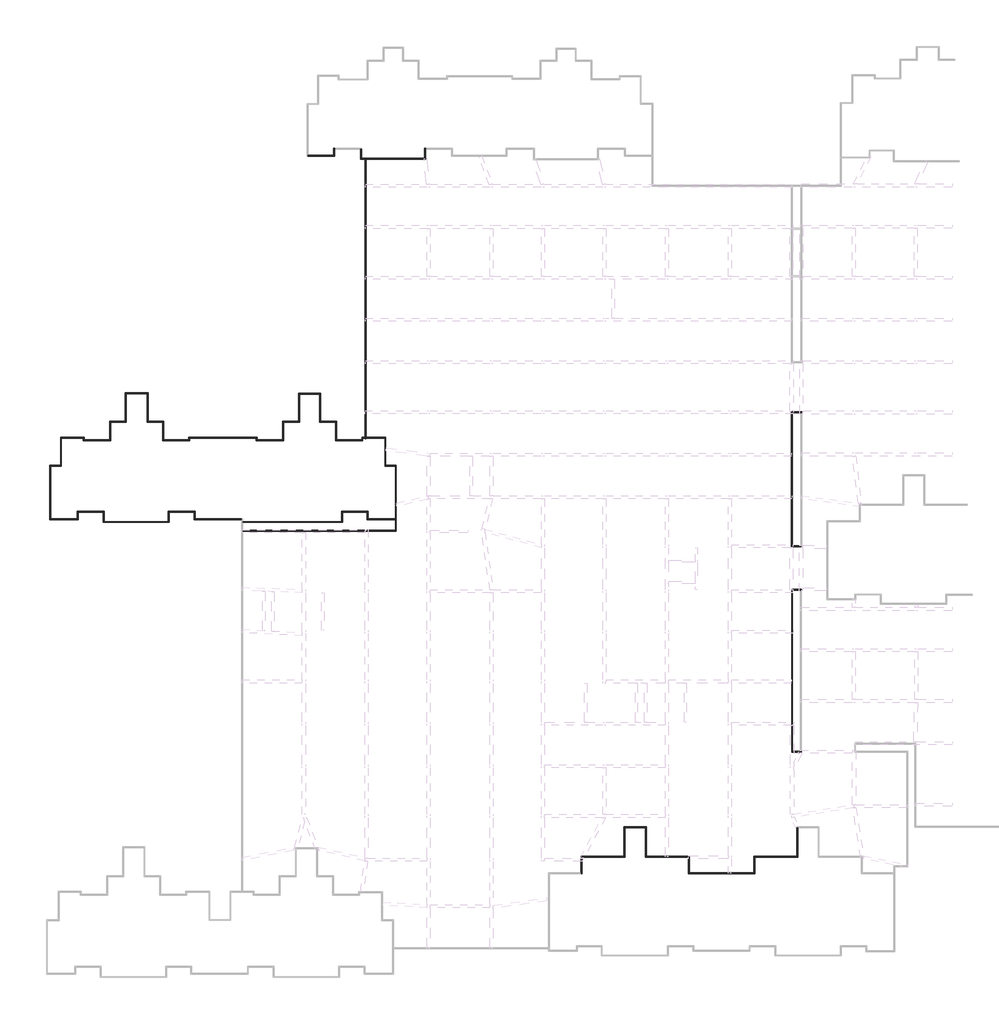
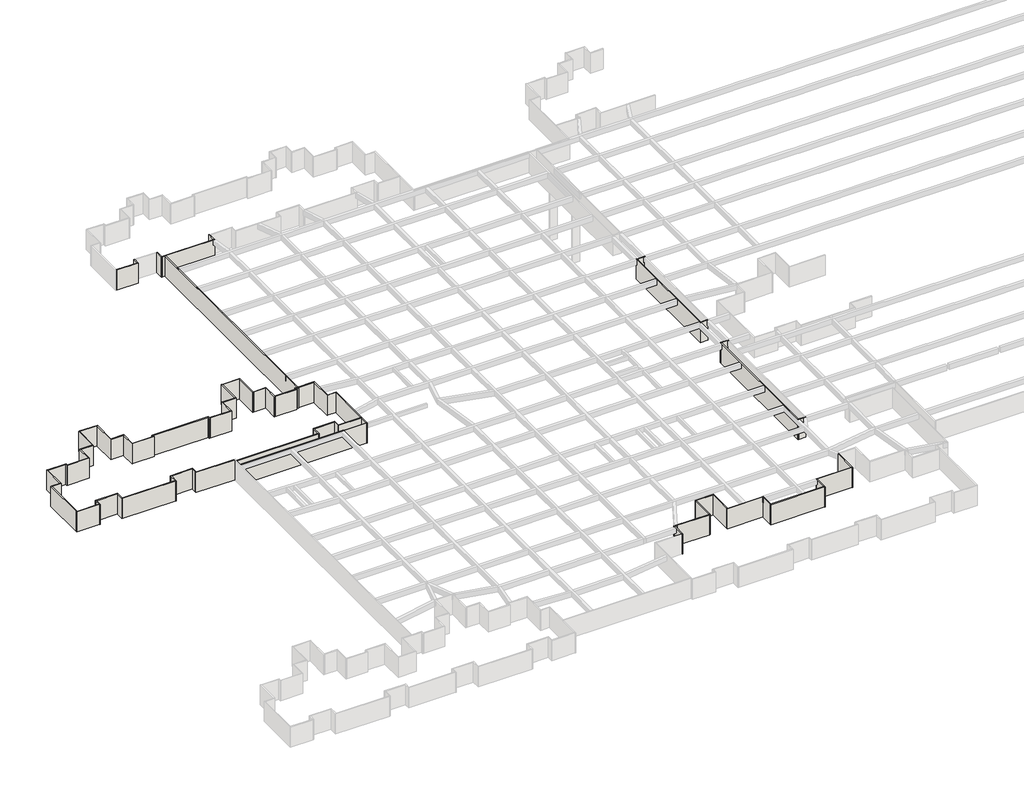
# One storey, part 2 of 16: 69 walls.
"""IFC4 building model written with IfcOpenShell, lengths in millimetres."""

from ifc_helpers import new_model, si_unit, origin, origin_with_axes, place, context, project, spatial, polyline, outline, extrude, faceted_brep, element, save

model = new_model("IFC4")

# Units and contexts
model_context = context("Model", 3, world=origin())
ifc_project = project(units=[si_unit("LENGTHUNIT", "METRE", prefix="MILLI")], contexts=[model_context])

# Site, building, storey
site = spatial("IfcSite", under=ifc_project)
building = spatial("IfcBuilding", under=site)
storey = spatial("IfcBuildingStorey", under=building, Name="户型图", Elevation=0.0)

# Walls
placement = place(None, origin())
element("IfcWall", 1, ObjectType="所有墙体", at=placement, inside=storey, context=model_context, shape_type="Brep", body=[
    faceted_brep([(192826.317546, -128736.151487, 0.0), (196226.317546, -128736.151487, 0.0), (196226.317546, -128736.151487, 3300.0), (192826.317546, -128736.151487, 3300.0), (192826.317546, -128616.151487, 0.0), (192826.317546, -128616.151487, 3300.0), (196106.317546, -128616.151487, 3300.0), (196226.317546, -128616.151487, 3300.0), (196226.317546, -128616.151487, 0.0), (196106.317546, -128616.151487, 0.0)], [[[0, 1, 2, 3]], [[4, 5, 6, 7, 8, 9]], [[1, 0, 4, 9, 8]], [[3, 2, 7, 6, 5]], [[0, 3, 5, 4]], [[2, 1, 8, 7]]]),
])
element("IfcWall", 2, ObjectType="所有墙体", at=placement, inside=storey, context=model_context, shape_type="Brep", body=[
    faceted_brep([(196226.317546, -128616.151487, 0.0), (196226.317546, -127836.151487, 0.0), (196226.317546, -127716.151487, 0.0), (196226.317546, -127716.151487, 3300.0), (196226.317546, -127836.151487, 3300.0), (196226.317546, -128616.151487, 3300.0), (196106.317546, -128616.151487, 0.0), (196106.317546, -128616.151487, 3300.0), (196106.317546, -127716.151487, 3300.0), (196106.317546, -127716.151487, 0.0)], [[[0, 1, 2, 3, 4, 5]], [[6, 7, 8, 9]], [[2, 1, 0, 6, 9]], [[5, 4, 3, 8, 7]], [[0, 5, 7, 6]], [[3, 2, 9, 8]]]),
])
element("IfcWall", 3, ObjectType="所有墙体", at=placement, inside=storey, context=model_context, shape_type="Brep", body=[
    faceted_brep([(199599.9062186, -127836.151487, 0.0), (199599.9062186, -129094.6769035, 0.0), (199599.9062186, -129094.6769035, 3300.0), (199599.9062186, -127836.151487, 3300.0), (199719.9062186, -127836.151487, 0.0), (199719.9062186, -127836.151487, 3300.0), (199719.9062186, -128974.6769035, 3300.0), (199719.9062186, -129094.6769035, 3300.0), (199719.9062186, -129094.6769035, 0.0), (199719.9062186, -128974.6769035, 0.0)], [[[0, 1, 2, 3]], [[4, 5, 6, 7, 8, 9]], [[1, 0, 4, 9, 8]], [[3, 2, 7, 6, 5]], [[0, 3, 5, 4]], [[2, 1, 8, 7]]]),
])
element("IfcWall", 4, ObjectType="所有墙体", at=placement, inside=storey, context=model_context, shape_type="Brep", body=[
    faceted_brep([(199719.9062186, -129094.6769035, 0.0), (200143.757676, -129094.6769035, 0.0), (200263.757676, -129094.6769035, 0.0), (207918.5069416, -129094.6769035, 0.0), (207918.5069416, -129094.6769035, 3300.0), (200263.757676, -129094.6769035, 3300.0), (200143.757676, -129094.6769035, 3300.0), (199719.9062186, -129094.6769035, 3300.0), (199719.9062186, -128974.6769035, 0.0), (199719.9062186, -128974.6769035, 3300.0), (207798.5069416, -128974.6769035, 3300.0), (207918.5069416, -128974.6769035, 3300.0), (207918.5069416, -128974.6769035, 0.0), (207798.5069416, -128974.6769035, 0.0)], [[[0, 1, 2, 3, 4, 5, 6, 7]], [[8, 9, 10, 11, 12, 13]], [[3, 2, 1, 0, 8, 13, 12]], [[7, 6, 5, 4, 11, 10, 9]], [[0, 7, 9, 8]], [[4, 3, 12, 11]]]),
])
element("IfcWall", 5, ObjectType="所有墙体", at=placement, inside=storey, context=model_context, shape_type="SweptSolid", body=[
    extrude(outline(polyline([(200143.757676, -165025.7214763), (200143.757676, -129094.6769035), (200263.757676, -129094.6769035), (200263.757676, -165025.7214763), (200143.757676, -165025.7214763)])), origin_with_axes(), (0.0, 0.0, 1.0), 3300.0),
])
element("IfcWall", 6, ObjectType="所有墙体", at=placement, inside=storey, context=model_context, shape_type="Brep", body=[
    faceted_brep([(207918.5069416, -128974.6769035, 0.0), (207918.5069416, -127836.151487, 0.0), (207918.5069416, -127716.151487, 0.0), (207918.5069416, -127716.151487, 3300.0), (207918.5069416, -127836.151487, 3300.0), (207918.5069416, -128974.6769035, 3300.0), (207798.5069416, -128974.6769035, 0.0), (207798.5069416, -128974.6769035, 3300.0), (207798.5069416, -127716.151487, 3300.0), (207798.5069416, -127716.151487, 0.0)], [[[0, 1, 2, 3, 4, 5]], [[6, 7, 8, 9]], [[2, 1, 0, 6, 9]], [[5, 4, 3, 8, 7]], [[0, 5, 7, 6]], [[3, 2, 9, 8]]]),
])
element("IfcWall", 7, ObjectType="所有墙体", at=placement, inside=storey, context=model_context, shape_type="Brep", body=[
    faceted_brep([(255612.4739458, -214925.8350287, 0.0), (255612.4739458, -218613.6358224, 0.0), (255612.4739458, -218733.6358224, 0.0), (255612.4739458, -218733.6358224, 3300.0), (255612.4739458, -218613.6358224, 3300.0), (255612.4739458, -214925.8350287, 3300.0), (255732.4739458, -214925.8350287, 0.0), (255732.4739458, -214925.8350287, 3300.0), (255732.4739458, -218733.6358224, 3300.0), (255732.4739458, -218733.6358224, 0.0)], [[[0, 1, 2, 3, 4, 5]], [[6, 7, 8, 9]], [[2, 1, 0, 6, 9]], [[5, 4, 3, 8, 7]], [[0, 5, 7, 6]], [[3, 2, 9, 8]]]),
])
element("IfcWall", 8, ObjectType="所有墙体", at=placement, inside=storey, context=model_context, shape_type="Brep", body=[
    faceted_brep([(255612.4739458, -218613.6358224, 0.0), (250108.5691963, -218613.6358224, 0.0), (250108.5691963, -218613.6358224, 3300.0), (255612.4739458, -218613.6358224, 3300.0), (255612.4739458, -218733.6358224, 0.0), (255612.4739458, -218733.6358224, 3300.0), (250228.5691963, -218733.6358224, 3300.0), (250108.5691963, -218733.6358224, 3300.0), (250108.5691963, -218733.6358224, 0.0), (250228.5691963, -218733.6358224, 0.0)], [[[0, 1, 2, 3]], [[4, 5, 6, 7, 8, 9]], [[1, 0, 4, 9, 8]], [[3, 2, 7, 6, 5]], [[0, 3, 5, 4]], [[2, 1, 8, 7]]]),
])
element("IfcWall", 9, ObjectType="所有墙体", at=placement, inside=storey, context=model_context, shape_type="Brep", body=[
    faceted_brep([(250108.5691963, -218733.6358224, 0.0), (250108.5691963, -220713.7545432, 0.0), (250108.5691963, -220833.7545432, 0.0), (250108.5691963, -220833.7545432, 3300.0), (250108.5691963, -220713.7545432, 3300.0), (250108.5691963, -218733.6358224, 3300.0), (250228.5691963, -218733.6358224, 0.0), (250228.5691963, -218733.6358224, 3300.0), (250228.5691963, -220833.7545432, 3300.0), (250228.5691963, -220833.7545432, 0.0)], [[[0, 1, 2, 3, 4, 5]], [[6, 7, 8, 9]], [[2, 1, 0, 6, 9]], [[5, 4, 3, 8, 7]], [[0, 5, 7, 6]], [[3, 2, 9, 8]]]),
])
element("IfcWall", 10, ObjectType="所有墙体", at=placement, inside=storey, context=model_context, shape_type="Brep", body=[
    faceted_brep([(250108.5691963, -220713.7545432, 0.0), (241826.9885063, -220713.7545432, 0.0), (241706.9885063, -220713.7545432, 0.0), (241706.9885063, -220713.7545432, 3300.0), (241826.9885063, -220713.7545432, 3300.0), (250108.5691963, -220713.7545432, 3300.0), (250108.5691963, -220833.7545432, 0.0), (250108.5691963, -220833.7545432, 3300.0), (241706.9885063, -220833.7545432, 3300.0), (241706.9885063, -220833.7545432, 0.0)], [[[0, 1, 2, 3, 4, 5]], [[6, 7, 8, 9]], [[2, 1, 0, 6, 9]], [[5, 4, 3, 8, 7]], [[0, 5, 7, 6]], [[3, 2, 9, 8]]]),
])
element("IfcWall", 11, ObjectType="所有墙体", at=placement, inside=storey, context=model_context, shape_type="Brep", body=[
    faceted_brep([(241826.9885063, -220713.7545432, 0.0), (241826.9885063, -218613.6358224, 0.0), (241826.9885063, -218613.6358224, 3300.0), (241826.9885063, -220713.7545432, 3300.0), (241706.9885063, -220713.7545432, 0.0), (241706.9885063, -220713.7545432, 3300.0), (241706.9885063, -218733.6358224, 3300.0), (241706.9885063, -218613.6358224, 3300.0), (241706.9885063, -218613.6358224, 0.0), (241706.9885063, -218733.6358224, 0.0)], [[[0, 1, 2, 3]], [[4, 5, 6, 7, 8, 9]], [[1, 0, 4, 9, 8]], [[3, 2, 7, 6, 5]], [[0, 3, 5, 4]], [[2, 1, 8, 7]]]),
])
element("IfcWall", 12, ObjectType="所有墙体", at=placement, inside=storey, context=model_context, shape_type="Brep", body=[
    faceted_brep([(241706.9885063, -218613.6358224, 0.0), (236279.3285625, -218613.6358224, 0.0), (236159.3285625, -218613.6358224, 0.0), (236159.3285625, -218613.6358224, 3300.0), (236279.3285625, -218613.6358224, 3300.0), (241706.9885063, -218613.6358224, 3300.0), (241706.9885063, -218733.6358224, 0.0), (241706.9885063, -218733.6358224, 3300.0), (236159.3285625, -218733.6358224, 3300.0), (236159.3285625, -218733.6358224, 0.0)], [[[0, 1, 2, 3, 4, 5]], [[6, 7, 8, 9]], [[2, 1, 0, 6, 9]], [[5, 4, 3, 8, 7]], [[0, 5, 7, 6]], [[3, 2, 9, 8]]]),
])
element("IfcWall", 13, ObjectType="所有墙体", at=placement, inside=storey, context=model_context, shape_type="Brep", body=[
    faceted_brep([(236279.3285625, -218613.6358224, 0.0), (236279.3285625, -214805.8350287, 0.0), (236279.3285625, -214805.8350287, 3300.0), (236279.3285625, -218613.6358224, 3300.0), (236159.3285625, -218613.6358224, 0.0), (236159.3285625, -218613.6358224, 3300.0), (236159.3285625, -214925.8350287, 3300.0), (236159.3285625, -214805.8350287, 3300.0), (236159.3285625, -214805.8350287, 0.0), (236159.3285625, -214925.8350287, 0.0)], [[[0, 1, 2, 3]], [[4, 5, 6, 7, 8, 9]], [[1, 0, 4, 9, 8]], [[3, 2, 7, 6, 5]], [[0, 3, 5, 4]], [[2, 1, 8, 7]]]),
])
element("IfcWall", 14, ObjectType="所有墙体", at=placement, inside=storey, context=model_context, shape_type="Brep", body=[
    faceted_brep([(236159.3285625, -214805.8350287, 0.0), (233412.4601239, -214805.8350287, 0.0), (233412.4601239, -214805.8350287, 3300.0), (236159.3285625, -214805.8350287, 3300.0), (236159.3285625, -214925.8350287, 0.0), (236159.3285625, -214925.8350287, 3300.0), (233532.4601239, -214925.8350287, 3300.0), (233412.4601239, -214925.8350287, 3300.0), (233412.4601239, -214925.8350287, 0.0), (233532.4601239, -214925.8350287, 0.0)], [[[0, 1, 2, 3]], [[4, 5, 6, 7, 8, 9]], [[1, 0, 4, 9, 8]], [[3, 2, 7, 6, 5]], [[0, 3, 5, 4]], [[2, 1, 8, 7]]]),
])
element("IfcWall", 15, ObjectType="所有墙体", at=placement, inside=storey, context=model_context, shape_type="Brep", body=[
    faceted_brep([(233412.4601239, -214925.8350287, 0.0), (233412.4601239, -218613.6358224, 0.0), (233412.4601239, -218733.6358224, 0.0), (233412.4601239, -218733.6358224, 3300.0), (233412.4601239, -218613.6358224, 3300.0), (233412.4601239, -214925.8350287, 3300.0), (233532.4601239, -214925.8350287, 0.0), (233532.4601239, -214925.8350287, 3300.0), (233532.4601239, -218733.6358224, 3300.0), (233532.4601239, -218733.6358224, 0.0)], [[[0, 1, 2, 3, 4, 5]], [[6, 7, 8, 9]], [[2, 1, 0, 6, 9]], [[5, 4, 3, 8, 7]], [[0, 5, 7, 6]], [[3, 2, 9, 8]]]),
])
element("IfcWall", 16, ObjectType="所有墙体", at=placement, inside=storey, context=model_context, shape_type="Brep", body=[
    faceted_brep([(233412.4601239, -218613.6358224, 0.0), (227909.4754658, -218613.6358224, 0.0), (227909.4754658, -218613.6358224, 3300.0), (233412.4601239, -218613.6358224, 3300.0), (233412.4601239, -218733.6358224, 0.0), (233412.4601239, -218733.6358224, 3300.0), (228029.4754658, -218733.6358224, 3300.0), (227909.4754658, -218733.6358224, 3300.0), (227909.4754658, -218733.6358224, 0.0), (228029.4754658, -218733.6358224, 0.0)], [[[0, 1, 2, 3]], [[4, 5, 6, 7, 8, 9]], [[1, 0, 4, 9, 8]], [[3, 2, 7, 6, 5]], [[0, 3, 5, 4]], [[2, 1, 8, 7]]]),
])
element("IfcWall", 17, ObjectType="所有墙体", at=placement, inside=storey, context=model_context, shape_type="Brep", body=[
    faceted_brep([(227909.4754658, -218733.6358224, 0.0), (227909.4754658, -220713.7545432, 0.0), (227909.4754658, -220833.7545432, 0.0), (227909.4754658, -220833.7545432, 3300.0), (227909.4754658, -220713.7545432, 3300.0), (227909.4754658, -218733.6358224, 3300.0), (228029.4754658, -218733.6358224, 0.0), (228029.4754658, -218733.6358224, 3300.0), (228029.4754658, -220833.7545432, 3300.0), (228029.4754658, -220833.7545432, 0.0)], [[[0, 1, 2, 3, 4, 5]], [[6, 7, 8, 9]], [[2, 1, 0, 6, 9]], [[5, 4, 3, 8, 7]], [[0, 5, 7, 6]], [[3, 2, 9, 8]]]),
])
element("IfcWall", 18, ObjectType="所有墙体", at=placement, inside=storey, context=model_context, shape_type="Brep", body=[
    faceted_brep([(184314.2189281, -175296.850594, 0.0), (178364.0035041, -175296.850594, 0.0), (178244.0035041, -175296.850594, 0.0), (178244.0035041, -175296.850594, 3300.0), (178364.0035041, -175296.850594, 3300.0), (184314.2189281, -175296.850594, 3300.0), (184314.2189281, -175416.850594, 0.0), (184314.2189281, -175416.850594, 3300.0), (178244.0035041, -175416.850594, 3300.0), (178244.0035041, -175416.850594, 0.0)], [[[0, 1, 2, 3, 4, 5]], [[6, 7, 8, 9]], [[2, 1, 0, 6, 9]], [[5, 4, 3, 8, 7]], [[0, 5, 7, 6]], [[3, 2, 9, 8]]]),
])
element("IfcWall", 19, ObjectType="所有墙体", at=placement, inside=storey, context=model_context, shape_type="Brep", body=[
    faceted_brep([(178364.0035041, -175296.850594, 0.0), (178364.0035041, -174337.1408994, 0.0), (178364.0035041, -174337.1408994, 3300.0), (178364.0035041, -175296.850594, 3300.0), (178244.0035041, -175296.850594, 0.0), (178244.0035041, -175296.850594, 3300.0), (178244.0035041, -174457.1408994, 3300.0), (178244.0035041, -174337.1408994, 3300.0), (178244.0035041, -174337.1408994, 0.0), (178244.0035041, -174457.1408994, 0.0)], [[[0, 1, 2, 3]], [[4, 5, 6, 7, 8, 9]], [[1, 0, 4, 9, 8]], [[3, 2, 7, 6, 5]], [[0, 3, 5, 4]], [[2, 1, 8, 7]]]),
])
element("IfcWall", 20, ObjectType="所有墙体", at=placement, inside=storey, context=model_context, shape_type="Brep", body=[
    faceted_brep([(178244.0035041, -174337.1408994, 0.0), (174893.4528763, -174337.1408994, 0.0), (174893.4528763, -174337.1408994, 3300.0), (178244.0035041, -174337.1408994, 3300.0), (178244.0035041, -174457.1408994, 0.0), (178244.0035041, -174457.1408994, 3300.0), (175013.4528763, -174457.1408994, 3300.0), (174893.4528763, -174457.1408994, 3300.0), (174893.4528763, -174457.1408994, 0.0), (175013.4528763, -174457.1408994, 0.0)], [[[0, 1, 2, 3]], [[4, 5, 6, 7, 8, 9]], [[1, 0, 4, 9, 8]], [[3, 2, 7, 6, 5]], [[0, 3, 5, 4]], [[2, 1, 8, 7]]]),
])
element("IfcWall", 21, ObjectType="所有墙体", at=placement, inside=storey, context=model_context, shape_type="Brep", body=[
    faceted_brep([(174893.4528763, -174457.1408994, 0.0), (174893.4528763, -175630.7737405, 0.0), (174893.4528763, -175750.7737405, 0.0), (174893.4528763, -175750.7737405, 3300.0), (174893.4528763, -175630.7737405, 3300.0), (174893.4528763, -174457.1408994, 3300.0), (175013.4528763, -174457.1408994, 0.0), (175013.4528763, -174457.1408994, 3300.0), (175013.4528763, -175750.7737405, 3300.0), (175013.4528763, -175750.7737405, 0.0)], [[[0, 1, 2, 3, 4, 5]], [[6, 7, 8, 9]], [[2, 1, 0, 6, 9]], [[5, 4, 3, 8, 7]], [[0, 5, 7, 6]], [[3, 2, 9, 8]]]),
])
element("IfcWall", 22, ObjectType="所有墙体", at=placement, inside=storey, context=model_context, shape_type="Brep", body=[
    faceted_brep([(174893.4528763, -175630.7737405, 0.0), (166663.6311033, -175630.7737405, 0.0), (166543.6311033, -175630.7737405, 0.0), (166543.6311033, -175630.7737405, 3300.0), (166663.6311033, -175630.7737405, 3300.0), (174893.4528763, -175630.7737405, 3300.0), (174893.4528763, -175750.7737405, 0.0), (174893.4528763, -175750.7737405, 3300.0), (166543.6311033, -175750.7737405, 3300.0), (166543.6311033, -175750.7737405, 0.0)], [[[0, 1, 2, 3, 4, 5]], [[6, 7, 8, 9]], [[2, 1, 0, 6, 9]], [[5, 4, 3, 8, 7]], [[0, 5, 7, 6]], [[3, 2, 9, 8]]]),
])
element("IfcWall", 23, ObjectType="所有墙体", at=placement, inside=storey, context=model_context, shape_type="Brep", body=[
    faceted_brep([(166663.6311033, -175630.7737405, 0.0), (166663.6311033, -174337.1408994, 0.0), (166663.6311033, -174337.1408994, 3300.0), (166663.6311033, -175630.7737405, 3300.0), (166543.6311033, -175630.7737405, 0.0), (166543.6311033, -175630.7737405, 3300.0), (166543.6311033, -174457.1408994, 3300.0), (166543.6311033, -174337.1408994, 3300.0), (166543.6311033, -174337.1408994, 0.0), (166543.6311033, -174457.1408994, 0.0)], [[[0, 1, 2, 3]], [[4, 5, 6, 7, 8, 9]], [[1, 0, 4, 9, 8]], [[3, 2, 7, 6, 5]], [[0, 3, 5, 4]], [[2, 1, 8, 7]]]),
])
element("IfcWall", 24, ObjectType="所有墙体", at=placement, inside=storey, context=model_context, shape_type="Brep", body=[
    faceted_brep([(166543.6311033, -174337.1408994, 0.0), (163193.621615, -174337.1408994, 0.0), (163193.621615, -174337.1408994, 3300.0), (166543.6311033, -174337.1408994, 3300.0), (166543.6311033, -174457.1408994, 0.0), (166543.6311033, -174457.1408994, 3300.0), (163313.621615, -174457.1408994, 3300.0), (163193.621615, -174457.1408994, 3300.0), (163193.621615, -174457.1408994, 0.0), (163313.621615, -174457.1408994, 0.0)], [[[0, 1, 2, 3]], [[4, 5, 6, 7, 8, 9]], [[1, 0, 4, 9, 8]], [[3, 2, 7, 6, 5]], [[0, 3, 5, 4]], [[2, 1, 8, 7]]]),
])
element("IfcWall", 25, ObjectType="所有墙体", at=placement, inside=storey, context=model_context, shape_type="Brep", body=[
    faceted_brep([(163193.621615, -174457.1408994, 0.0), (163193.621615, -175296.850594, 0.0), (163193.621615, -175416.850594, 0.0), (163193.621615, -175416.850594, 3300.0), (163193.621615, -175296.850594, 3300.0), (163193.621615, -174457.1408994, 3300.0), (163313.621615, -174457.1408994, 0.0), (163313.621615, -174457.1408994, 3300.0), (163313.621615, -175416.850594, 3300.0), (163313.621615, -175416.850594, 0.0)], [[[0, 1, 2, 3, 4, 5]], [[6, 7, 8, 9]], [[2, 1, 0, 6, 9]], [[5, 4, 3, 8, 7]], [[0, 5, 7, 6]], [[3, 2, 9, 8]]]),
])
element("IfcWall", 26, ObjectType="所有墙体", at=placement, inside=storey, context=model_context, shape_type="Brep", body=[
    faceted_brep([(163193.621615, -175296.850594, 0.0), (159761.9565395, -175296.850594, 0.0), (159641.9565395, -175296.850594, 0.0), (159641.9565395, -175296.850594, 3300.0), (159761.9565395, -175296.850594, 3300.0), (163193.621615, -175296.850594, 3300.0), (163193.621615, -175416.850594, 0.0), (163193.621615, -175416.850594, 3300.0), (159641.9565395, -175416.850594, 3300.0), (159641.9565395, -175416.850594, 0.0)], [[[0, 1, 2, 3, 4, 5]], [[6, 7, 8, 9]], [[2, 1, 0, 6, 9]], [[5, 4, 3, 8, 7]], [[0, 5, 7, 6]], [[3, 2, 9, 8]]]),
])
element("IfcWall", 27, ObjectType="所有墙体", at=placement, inside=storey, context=model_context, shape_type="Brep", body=[
    faceted_brep([(159761.9565395, -175296.850594, 0.0), (159761.9565395, -168538.1791139, 0.0), (159761.9565395, -168418.1791139, 0.0), (159761.9565395, -168418.1791139, 3300.0), (159761.9565395, -168538.1791139, 3300.0), (159761.9565395, -175296.850594, 3300.0), (159641.9565395, -175296.850594, 0.0), (159641.9565395, -175296.850594, 3300.0), (159641.9565395, -168418.1791139, 3300.0), (159641.9565395, -168418.1791139, 0.0)], [[[0, 1, 2, 3, 4, 5]], [[6, 7, 8, 9]], [[2, 1, 0, 6, 9]], [[5, 4, 3, 8, 7]], [[0, 5, 7, 6]], [[3, 2, 9, 8]]]),
])
element("IfcWall", 28, ObjectType="所有墙体", at=placement, inside=storey, context=model_context, shape_type="Brep", body=[
    faceted_brep([(159761.9565395, -168538.1791139, 0.0), (161173.1931827, -168538.1791139, 0.0), (161173.1931827, -168538.1791139, 3300.0), (159761.9565395, -168538.1791139, 3300.0), (159761.9565395, -168418.1791139, 0.0), (159761.9565395, -168418.1791139, 3300.0), (161053.1931827, -168418.1791139, 3300.0), (161173.1931827, -168418.1791139, 3300.0), (161173.1931827, -168418.1791139, 0.0), (161053.1931827, -168418.1791139, 0.0)], [[[0, 1, 2, 3]], [[4, 5, 6, 7, 8, 9]], [[1, 0, 4, 9, 8]], [[3, 2, 7, 6, 5]], [[0, 3, 5, 4]], [[2, 1, 8, 7]]]),
])
element("IfcWall", 29, ObjectType="所有墙体", at=placement, inside=storey, context=model_context, shape_type="Brep", body=[
    faceted_brep([(161173.1931827, -168418.1791139, 0.0), (161173.1931827, -164940.1944172, 0.0), (161173.1931827, -164820.1944172, 0.0), (161173.1931827, -164820.1944172, 3300.0), (161173.1931827, -164940.1944172, 3300.0), (161173.1931827, -168418.1791139, 3300.0), (161053.1931827, -168418.1791139, 0.0), (161053.1931827, -168418.1791139, 3300.0), (161053.1931827, -164820.1944172, 3300.0), (161053.1931827, -164820.1944172, 0.0)], [[[0, 1, 2, 3, 4, 5]], [[6, 7, 8, 9]], [[2, 1, 0, 6, 9]], [[5, 4, 3, 8, 7]], [[0, 5, 7, 6]], [[3, 2, 9, 8]]]),
])
element("IfcWall", 30, ObjectType="所有墙体", at=placement, inside=storey, context=model_context, shape_type="Brep", body=[
    faceted_brep([(161173.1931827, -164940.1944172, 0.0), (163955.0209252, -164940.1944172, 0.0), (164075.0209252, -164940.1944172, 0.0), (164075.0209252, -164940.1944172, 3300.0), (163955.0209252, -164940.1944172, 3300.0), (161173.1931827, -164940.1944172, 3300.0), (161173.1931827, -164820.1944172, 0.0), (161173.1931827, -164820.1944172, 3300.0), (164075.0209252, -164820.1944172, 3300.0), (164075.0209252, -164820.1944172, 0.0)], [[[0, 1, 2, 3, 4, 5]], [[6, 7, 8, 9]], [[2, 1, 0, 6, 9]], [[5, 4, 3, 8, 7]], [[0, 5, 7, 6]], [[3, 2, 9, 8]]]),
])
element("IfcWall", 31, ObjectType="所有墙体", at=placement, inside=storey, context=model_context, shape_type="Brep", body=[
    faceted_brep([(163955.0209252, -164940.1944172, 0.0), (163955.0209252, -165244.2945353, 0.0), (163955.0209252, -165244.2945353, 3300.0), (163955.0209252, -164940.1944172, 3300.0), (164075.0209252, -164940.1944172, 0.0), (164075.0209252, -164940.1944172, 3300.0), (164075.0209252, -165124.2945353, 3300.0), (164075.0209252, -165244.2945353, 3300.0), (164075.0209252, -165244.2945353, 0.0), (164075.0209252, -165124.2945353, 0.0)], [[[0, 1, 2, 3]], [[4, 5, 6, 7, 8, 9]], [[1, 0, 4, 9, 8]], [[3, 2, 7, 6, 5]], [[0, 3, 5, 4]], [[2, 1, 8, 7]]]),
])
element("IfcWall", 32, ObjectType="所有墙体", at=placement, inside=storey, context=model_context, shape_type="Brep", body=[
    faceted_brep([(164075.0209252, -165244.2945353, 0.0), (167477.7279266, -165244.2945353, 0.0), (167477.7279266, -165244.2945353, 3300.0), (164075.0209252, -165244.2945353, 3300.0), (164075.0209252, -165124.2945353, 0.0), (164075.0209252, -165124.2945353, 3300.0), (167357.7279266, -165124.2945353, 3300.0), (167477.7279266, -165124.2945353, 3300.0), (167477.7279266, -165124.2945353, 0.0), (167357.7279266, -165124.2945353, 0.0)], [[[0, 1, 2, 3]], [[4, 5, 6, 7, 8, 9]], [[1, 0, 4, 9, 8]], [[3, 2, 7, 6, 5]], [[0, 3, 5, 4]], [[2, 1, 8, 7]]]),
])
element("IfcWall", 33, ObjectType="所有墙体", at=placement, inside=storey, context=model_context, shape_type="Brep", body=[
    faceted_brep([(167477.7279266, -165124.2945353, 0.0), (167477.7279266, -162896.0646856, 0.0), (167477.7279266, -162776.0646856, 0.0), (167477.7279266, -162776.0646856, 3300.0), (167477.7279266, -162896.0646856, 3300.0), (167477.7279266, -165124.2945353, 3300.0), (167357.7279266, -165124.2945353, 0.0), (167357.7279266, -165124.2945353, 3300.0), (167357.7279266, -162776.0646856, 3300.0), (167357.7279266, -162776.0646856, 0.0)], [[[0, 1, 2, 3, 4, 5]], [[6, 7, 8, 9]], [[2, 1, 0, 6, 9]], [[5, 4, 3, 8, 7]], [[0, 5, 7, 6]], [[3, 2, 9, 8]]]),
])
element("IfcWall", 34, ObjectType="所有墙体", at=placement, inside=storey, context=model_context, shape_type="Brep", body=[
    faceted_brep([(167477.7279266, -162896.0646856, 0.0), (169482.0893919, -162896.0646856, 0.0), (169482.0893919, -162896.0646856, 3300.0), (167477.7279266, -162896.0646856, 3300.0), (167477.7279266, -162776.0646856, 0.0), (167477.7279266, -162776.0646856, 3300.0), (169362.0893919, -162776.0646856, 3300.0), (169482.0893919, -162776.0646856, 3300.0), (169482.0893919, -162776.0646856, 0.0), (169362.0893919, -162776.0646856, 0.0)], [[[0, 1, 2, 3]], [[4, 5, 6, 7, 8, 9]], [[1, 0, 4, 9, 8]], [[3, 2, 7, 6, 5]], [[0, 3, 5, 4]], [[2, 1, 8, 7]]]),
])
element("IfcWall", 35, ObjectType="所有墙体", at=placement, inside=storey, context=model_context, shape_type="Brep", body=[
    faceted_brep([(169482.0893919, -162776.0646856, 0.0), (169482.0893919, -159200.6661517, 0.0), (169482.0893919, -159080.6661517, 0.0), (169482.0893919, -159080.6661517, 3300.0), (169482.0893919, -159200.6661517, 3300.0), (169482.0893919, -162776.0646856, 3300.0), (169362.0893919, -162776.0646856, 0.0), (169362.0893919, -162776.0646856, 3300.0), (169362.0893919, -159080.6661517, 3300.0), (169362.0893919, -159080.6661517, 0.0)], [[[0, 1, 2, 3, 4, 5]], [[6, 7, 8, 9]], [[2, 1, 0, 6, 9]], [[5, 4, 3, 8, 7]], [[0, 5, 7, 6]], [[3, 2, 9, 8]]]),
])
element("IfcWall", 36, ObjectType="所有墙体", at=placement, inside=storey, context=model_context, shape_type="Brep", body=[
    faceted_brep([(169482.0893919, -159200.6661517, 0.0), (172157.72459, -159200.6661517, 0.0), (172277.72459, -159200.6661517, 0.0), (172277.72459, -159200.6661517, 3300.0), (172157.72459, -159200.6661517, 3300.0), (169482.0893919, -159200.6661517, 3300.0), (169482.0893919, -159080.6661517, 0.0), (169482.0893919, -159080.6661517, 3300.0), (172277.72459, -159080.6661517, 3300.0), (172277.72459, -159080.6661517, 0.0)], [[[0, 1, 2, 3, 4, 5]], [[6, 7, 8, 9]], [[2, 1, 0, 6, 9]], [[5, 4, 3, 8, 7]], [[0, 5, 7, 6]], [[3, 2, 9, 8]]]),
])
element("IfcWall", 37, ObjectType="所有墙体", at=placement, inside=storey, context=model_context, shape_type="Brep", body=[
    faceted_brep([(172157.72459, -159200.6661517, 0.0), (172157.72459, -162896.0646856, 0.0), (172157.72459, -162896.0646856, 3300.0), (172157.72459, -159200.6661517, 3300.0), (172277.72459, -159200.6661517, 0.0), (172277.72459, -159200.6661517, 3300.0), (172277.72459, -162776.0646856, 3300.0), (172277.72459, -162896.0646856, 3300.0), (172277.72459, -162896.0646856, 0.0), (172277.72459, -162776.0646856, 0.0)], [[[0, 1, 2, 3]], [[4, 5, 6, 7, 8, 9]], [[1, 0, 4, 9, 8]], [[3, 2, 7, 6, 5]], [[0, 3, 5, 4]], [[2, 1, 8, 7]]]),
])
element("IfcWall", 38, ObjectType="所有墙体", at=placement, inside=storey, context=model_context, shape_type="Brep", body=[
    faceted_brep([(172277.72459, -162896.0646856, 0.0), (174156.2592036, -162896.0646856, 0.0), (174276.2592036, -162896.0646856, 0.0), (174276.2592036, -162896.0646856, 3300.0), (174156.2592036, -162896.0646856, 3300.0), (172277.72459, -162896.0646856, 3300.0), (172277.72459, -162776.0646856, 0.0), (172277.72459, -162776.0646856, 3300.0), (174276.2592036, -162776.0646856, 3300.0), (174276.2592036, -162776.0646856, 0.0)], [[[0, 1, 2, 3, 4, 5]], [[6, 7, 8, 9]], [[2, 1, 0, 6, 9]], [[5, 4, 3, 8, 7]], [[0, 5, 7, 6]], [[3, 2, 9, 8]]]),
])
element("IfcWall", 39, ObjectType="所有墙体", at=placement, inside=storey, context=model_context, shape_type="Brep", body=[
    faceted_brep([(174156.2592036, -162896.0646856, 0.0), (174156.2592036, -165244.2945353, 0.0), (174156.2592036, -165244.2945353, 3300.0), (174156.2592036, -162896.0646856, 3300.0), (174276.2592036, -162896.0646856, 0.0), (174276.2592036, -162896.0646856, 3300.0), (174276.2592036, -165124.2945353, 3300.0), (174276.2592036, -165244.2945353, 3300.0), (174276.2592036, -165244.2945353, 0.0), (174276.2592036, -165124.2945353, 0.0)], [[[0, 1, 2, 3]], [[4, 5, 6, 7, 8, 9]], [[1, 0, 4, 9, 8]], [[3, 2, 7, 6, 5]], [[0, 3, 5, 4]], [[2, 1, 8, 7]]]),
])
element("IfcWall", 40, ObjectType="所有墙体", at=placement, inside=storey, context=model_context, shape_type="Brep", body=[
    faceted_brep([(174276.2592036, -165244.2945353, 0.0), (177625.6147377, -165244.2945353, 0.0), (177625.6147377, -165244.2945353, 3300.0), (174276.2592036, -165244.2945353, 3300.0), (174276.2592036, -165124.2945353, 0.0), (174276.2592036, -165124.2945353, 3300.0), (177505.6147377, -165124.2945353, 3300.0), (177625.6147377, -165124.2945353, 3300.0), (177625.6147377, -165124.2945353, 0.0), (177505.6147377, -165124.2945353, 0.0)], [[[0, 1, 2, 3]], [[4, 5, 6, 7, 8, 9]], [[1, 0, 4, 9, 8]], [[3, 2, 7, 6, 5]], [[0, 3, 5, 4]], [[2, 1, 8, 7]]]),
])
element("IfcWall", 41, ObjectType="所有墙体", at=placement, inside=storey, context=model_context, shape_type="Brep", body=[
    faceted_brep([(177625.6147377, -165124.2945353, 0.0), (177625.6147377, -164940.1944172, 0.0), (177625.6147377, -164820.1944172, 0.0), (177625.6147377, -164820.1944172, 3300.0), (177625.6147377, -164940.1944172, 3300.0), (177625.6147377, -165124.2945353, 3300.0), (177505.6147377, -165124.2945353, 0.0), (177505.6147377, -165124.2945353, 3300.0), (177505.6147377, -164820.1944172, 3300.0), (177505.6147377, -164820.1944172, 0.0)], [[[0, 1, 2, 3, 4, 5]], [[6, 7, 8, 9]], [[2, 1, 0, 6, 9]], [[5, 4, 3, 8, 7]], [[0, 5, 7, 6]], [[3, 2, 9, 8]]]),
])
element("IfcWall", 42, ObjectType="所有墙体", at=placement, inside=storey, context=model_context, shape_type="Brep", body=[
    faceted_brep([(177625.6147377, -164940.1944172, 0.0), (186205.0363238, -164940.1944172, 0.0), (186325.0363238, -164940.1944172, 0.0), (186325.0363238, -164940.1944172, 3300.0), (186205.0363238, -164940.1944172, 3300.0), (177625.6147377, -164940.1944172, 3300.0), (177625.6147377, -164820.1944172, 0.0), (177625.6147377, -164820.1944172, 3300.0), (186325.0363238, -164820.1944172, 3300.0), (186325.0363238, -164820.1944172, 0.0)], [[[0, 1, 2, 3, 4, 5]], [[6, 7, 8, 9]], [[2, 1, 0, 6, 9]], [[5, 4, 3, 8, 7]], [[0, 5, 7, 6]], [[3, 2, 9, 8]]]),
])
element("IfcWall", 43, ObjectType="所有墙体", at=placement, inside=storey, context=model_context, shape_type="Brep", body=[
    faceted_brep([(186205.0363238, -164940.1944172, 0.0), (186205.0363238, -165244.2945353, 0.0), (186205.0363238, -165244.2945353, 3300.0), (186205.0363238, -164940.1944172, 3300.0), (186325.0363238, -164940.1944172, 0.0), (186325.0363238, -164940.1944172, 3300.0), (186325.0363238, -165124.2945353, 3300.0), (186325.0363238, -165244.2945353, 3300.0), (186325.0363238, -165244.2945353, 0.0), (186325.0363238, -165124.2945353, 0.0)], [[[0, 1, 2, 3]], [[4, 5, 6, 7, 8, 9]], [[1, 0, 4, 9, 8]], [[3, 2, 7, 6, 5]], [[0, 3, 5, 4]], [[2, 1, 8, 7]]]),
])
element("IfcWall", 44, ObjectType="所有墙体", at=placement, inside=storey, context=model_context, shape_type="Brep", body=[
    faceted_brep([(186325.0363238, -165244.2945353, 0.0), (189677.7124936, -165244.2945353, 0.0), (189677.7124936, -165244.2945353, 3300.0), (186325.0363238, -165244.2945353, 3300.0), (186325.0363238, -165124.2945353, 0.0), (186325.0363238, -165124.2945353, 3300.0), (189557.7124936, -165124.2945353, 3300.0), (189677.7124936, -165124.2945353, 3300.0), (189677.7124936, -165124.2945353, 0.0), (189557.7124936, -165124.2945353, 0.0)], [[[0, 1, 2, 3]], [[4, 5, 6, 7, 8, 9]], [[1, 0, 4, 9, 8]], [[3, 2, 7, 6, 5]], [[0, 3, 5, 4]], [[2, 1, 8, 7]]]),
])
element("IfcWall", 45, ObjectType="所有墙体", at=placement, inside=storey, context=model_context, shape_type="Brep", body=[
    faceted_brep([(189677.7124936, -165124.2945353, 0.0), (189677.7124936, -162896.0646856, 0.0), (189677.7124936, -162776.0646856, 0.0), (189677.7124936, -162776.0646856, 3300.0), (189677.7124936, -162896.0646856, 3300.0), (189677.7124936, -165124.2945353, 3300.0), (189557.7124936, -165124.2945353, 0.0), (189557.7124936, -165124.2945353, 3300.0), (189557.7124936, -162776.0646856, 3300.0), (189557.7124936, -162776.0646856, 0.0)], [[[0, 1, 2, 3, 4, 5]], [[6, 7, 8, 9]], [[2, 1, 0, 6, 9]], [[5, 4, 3, 8, 7]], [[0, 5, 7, 6]], [[3, 2, 9, 8]]]),
])
element("IfcWall", 46, ObjectType="所有墙体", at=placement, inside=storey, context=model_context, shape_type="Brep", body=[
    faceted_brep([(189677.7124936, -162896.0646856, 0.0), (191731.2823751, -162896.0646856, 0.0), (191731.2823751, -162896.0646856, 3300.0), (189677.7124936, -162896.0646856, 3300.0), (189677.7124936, -162776.0646856, 0.0), (189677.7124936, -162776.0646856, 3300.0), (191611.2823751, -162776.0646856, 3300.0), (191731.2823751, -162776.0646856, 3300.0), (191731.2823751, -162776.0646856, 0.0), (191611.2823751, -162776.0646856, 0.0)], [[[0, 1, 2, 3]], [[4, 5, 6, 7, 8, 9]], [[1, 0, 4, 9, 8]], [[3, 2, 7, 6, 5]], [[0, 3, 5, 4]], [[2, 1, 8, 7]]]),
])
element("IfcWall", 47, ObjectType="所有墙体", at=placement, inside=storey, context=model_context, shape_type="Brep", body=[
    faceted_brep([(191731.2823751, -162776.0646856, 0.0), (191731.2823751, -159278.1403142, 0.0), (191731.2823751, -159158.1403142, 0.0), (191731.2823751, -159158.1403142, 3300.0), (191731.2823751, -159278.1403142, 3300.0), (191731.2823751, -162776.0646856, 3300.0), (191611.2823751, -162776.0646856, 0.0), (191611.2823751, -162776.0646856, 3300.0), (191611.2823751, -159158.1403142, 3300.0), (191611.2823751, -159158.1403142, 0.0)], [[[0, 1, 2, 3, 4, 5]], [[6, 7, 8, 9]], [[2, 1, 0, 6, 9]], [[5, 4, 3, 8, 7]], [[0, 5, 7, 6]], [[3, 2, 9, 8]]]),
])
element("IfcWall", 48, ObjectType="所有墙体", at=placement, inside=storey, context=model_context, shape_type="Brep", body=[
    faceted_brep([(191731.2823751, -159278.1403142, 0.0), (194357.7091566, -159278.1403142, 0.0), (194477.7091566, -159278.1403142, 0.0), (194477.7091566, -159278.1403142, 3300.0), (194357.7091566, -159278.1403142, 3300.0), (191731.2823751, -159278.1403142, 3300.0), (191731.2823751, -159158.1403142, 0.0), (191731.2823751, -159158.1403142, 3300.0), (194477.7091566, -159158.1403142, 3300.0), (194477.7091566, -159158.1403142, 0.0)], [[[0, 1, 2, 3, 4, 5]], [[6, 7, 8, 9]], [[2, 1, 0, 6, 9]], [[5, 4, 3, 8, 7]], [[0, 5, 7, 6]], [[3, 2, 9, 8]]]),
])
element("IfcWall", 49, ObjectType="所有墙体", at=placement, inside=storey, context=model_context, shape_type="Brep", body=[
    faceted_brep([(194357.7091566, -159278.1403142, 0.0), (194357.7091566, -162896.0646856, 0.0), (194357.7091566, -162896.0646856, 3300.0), (194357.7091566, -159278.1403142, 3300.0), (194477.7091566, -159278.1403142, 0.0), (194477.7091566, -159278.1403142, 3300.0), (194477.7091566, -162776.0646856, 3300.0), (194477.7091566, -162896.0646856, 3300.0), (194477.7091566, -162896.0646856, 0.0), (194477.7091566, -162776.0646856, 0.0)], [[[0, 1, 2, 3]], [[4, 5, 6, 7, 8, 9]], [[1, 0, 4, 9, 8]], [[3, 2, 7, 6, 5]], [[0, 3, 5, 4]], [[2, 1, 8, 7]]]),
])
element("IfcWall", 50, ObjectType="所有墙体", at=placement, inside=storey, context=model_context, shape_type="Brep", body=[
    faceted_brep([(194477.7091566, -162896.0646856, 0.0), (196356.274637, -162896.0646856, 0.0), (196476.274637, -162896.0646856, 0.0), (196476.274637, -162896.0646856, 3300.0), (196356.274637, -162896.0646856, 3300.0), (194477.7091566, -162896.0646856, 3300.0), (194477.7091566, -162776.0646856, 0.0), (194477.7091566, -162776.0646856, 3300.0), (196476.274637, -162776.0646856, 3300.0), (196476.274637, -162776.0646856, 0.0)], [[[0, 1, 2, 3, 4, 5]], [[6, 7, 8, 9]], [[2, 1, 0, 6, 9]], [[5, 4, 3, 8, 7]], [[0, 5, 7, 6]], [[3, 2, 9, 8]]]),
])
element("IfcWall", 51, ObjectType="所有墙体", at=placement, inside=storey, context=model_context, shape_type="Brep", body=[
    faceted_brep([(196356.274637, -162896.0646856, 0.0), (196356.274637, -165244.2945353, 0.0), (196356.274637, -165244.2945353, 3300.0), (196356.274637, -162896.0646856, 3300.0), (196476.274637, -162896.0646856, 0.0), (196476.274637, -162896.0646856, 3300.0), (196476.274637, -165124.2945353, 3300.0), (196476.274637, -165244.2945353, 3300.0), (196476.274637, -165244.2945353, 0.0), (196476.274637, -165124.2945353, 0.0)], [[[0, 1, 2, 3]], [[4, 5, 6, 7, 8, 9]], [[1, 0, 4, 9, 8]], [[3, 2, 7, 6, 5]], [[0, 3, 5, 4]], [[2, 1, 8, 7]]]),
])
element("IfcWall", 52, ObjectType="所有墙体", at=placement, inside=storey, context=model_context, shape_type="Brep", body=[
    faceted_brep([(196476.274637, -165244.2945353, 0.0), (199875.0405613, -165244.2945353, 0.0), (199875.0405613, -165244.2945353, 3300.0), (196476.274637, -165244.2945353, 3300.0), (196476.274637, -165124.2945353, 0.0), (196476.274637, -165124.2945353, 3300.0), (199755.0405613, -165124.2945353, 3300.0), (199875.0405613, -165124.2945353, 3300.0), (199875.0405613, -165124.2945353, 0.0), (199755.0405613, -165124.2945353, 0.0)], [[[0, 1, 2, 3]], [[4, 5, 6, 7, 8, 9]], [[1, 0, 4, 9, 8]], [[3, 2, 7, 6, 5]], [[0, 3, 5, 4]], [[2, 1, 8, 7]]]),
])
element("IfcWall", 53, ObjectType="所有墙体", at=placement, inside=storey, context=model_context, shape_type="Brep", body=[
    faceted_brep([(199875.0405613, -165124.2945353, 0.0), (199875.0405613, -164940.1944172, 0.0), (199875.0405613, -164820.1944172, 0.0), (199875.0405613, -164820.1944172, 3300.0), (199875.0405613, -164940.1944172, 3300.0), (199875.0405613, -165124.2945353, 3300.0), (199755.0405613, -165124.2945353, 0.0), (199755.0405613, -165124.2945353, 3300.0), (199755.0405613, -164820.1944172, 3300.0), (199755.0405613, -164820.1944172, 0.0)], [[[0, 1, 2, 3, 4, 5]], [[6, 7, 8, 9]], [[2, 1, 0, 6, 9]], [[5, 4, 3, 8, 7]], [[0, 5, 7, 6]], [[3, 2, 9, 8]]]),
])
element("IfcWall", 54, ObjectType="所有墙体", at=placement, inside=storey, context=model_context, shape_type="Brep", body=[
    faceted_brep([(199875.0405613, -164940.1944172, 0.0), (202705.4014006, -164940.1944172, 0.0), (202825.4014006, -164940.1944172, 0.0), (202825.4014006, -164940.1944172, 3300.0), (202705.4014006, -164940.1944172, 3300.0), (199875.0405613, -164940.1944172, 3300.0), (199875.0405613, -164820.1944172, 0.0), (199875.0405613, -164820.1944172, 3300.0), (202825.4014006, -164820.1944172, 3300.0), (202825.4014006, -164820.1944172, 0.0)], [[[0, 1, 2, 3, 4, 5]], [[6, 7, 8, 9]], [[2, 1, 0, 6, 9]], [[5, 4, 3, 8, 7]], [[0, 5, 7, 6]], [[3, 2, 9, 8]]]),
])
element("IfcWall", 55, ObjectType="所有墙体", at=placement, inside=storey, context=model_context, shape_type="Brep", body=[
    faceted_brep([(202705.4014006, -164940.1944172, 0.0), (202705.4014006, -168537.9797868, 0.0), (202705.4014006, -168537.9797868, 3300.0), (202705.4014006, -164940.1944172, 3300.0), (202825.4014006, -164940.1944172, 0.0), (202825.4014006, -164940.1944172, 3300.0), (202825.4014006, -168417.9797868, 3300.0), (202825.4014006, -168537.9797868, 3300.0), (202825.4014006, -168537.9797868, 0.0), (202825.4014006, -168417.9797868, 0.0)], [[[0, 1, 2, 3]], [[4, 5, 6, 7, 8, 9]], [[1, 0, 4, 9, 8]], [[3, 2, 7, 6, 5]], [[0, 3, 5, 4]], [[2, 1, 8, 7]]]),
])
element("IfcWall", 56, ObjectType="所有墙体", at=placement, inside=storey, context=model_context, shape_type="Brep", body=[
    faceted_brep([(202825.4014006, -168537.9797868, 0.0), (204051.1600072, -168537.9797868, 0.0), (204171.1600072, -168537.9797868, 0.0), (204171.1600072, -168537.9797868, 3300.0), (204051.1600072, -168537.9797868, 3300.0), (202825.4014006, -168537.9797868, 3300.0), (202825.4014006, -168417.9797868, 0.0), (202825.4014006, -168417.9797868, 3300.0), (204171.1600072, -168417.9797868, 3300.0), (204171.1600072, -168417.9797868, 0.0)], [[[0, 1, 2, 3, 4, 5]], [[6, 7, 8, 9]], [[2, 1, 0, 6, 9]], [[5, 4, 3, 8, 7]], [[0, 5, 7, 6]], [[3, 2, 9, 8]]]),
])
element("IfcWall", 57, ObjectType="所有墙体", at=placement, inside=storey, context=model_context, shape_type="Brep", body=[
    faceted_brep([(204051.1600072, -168537.9797868, 0.0), (204051.1600072, -175296.850594, 0.0), (204051.1600072, -175416.850594, 0.0), (204051.1600072, -176745.1471774, 0.0), (204051.1600072, -176865.1471774, 0.0), (204051.1600072, -176865.1471774, 3300.0), (204051.1600072, -176745.1471774, 3300.0), (204051.1600072, -175416.850594, 3300.0), (204051.1600072, -175296.850594, 3300.0), (204051.1600072, -168537.9797868, 3300.0), (204171.1600072, -168537.9797868, 0.0), (204171.1600072, -168537.9797868, 3300.0), (204171.1600072, -176865.1471774, 3300.0), (204171.1600072, -176865.1471774, 0.0)], [[[0, 1, 2, 3, 4, 5, 6, 7, 8, 9]], [[10, 11, 12, 13]], [[4, 3, 2, 1, 0, 10, 13]], [[9, 8, 7, 6, 5, 12, 11]], [[0, 9, 11, 10]], [[5, 4, 13, 12]]]),
])
element("IfcWall", 58, ObjectType="所有墙体", at=placement, inside=storey, context=model_context, shape_type="Brep", body=[
    faceted_brep([(204051.1600072, -175296.850594, 0.0), (200563.757676, -175296.850594, 0.0), (200443.757676, -175296.850594, 0.0), (200443.757676, -175296.850594, 3300.0), (200563.757676, -175296.850594, 3300.0), (204051.1600072, -175296.850594, 3300.0), (204051.1600072, -175416.850594, 0.0), (204051.1600072, -175416.850594, 3300.0), (200443.757676, -175416.850594, 3300.0), (200443.757676, -175416.850594, 0.0)], [[[0, 1, 2, 3, 4, 5]], [[6, 7, 8, 9]], [[2, 1, 0, 6, 9]], [[5, 4, 3, 8, 7]], [[0, 5, 7, 6]], [[3, 2, 9, 8]]]),
])
element("IfcWall", 59, ObjectType="所有墙体", at=placement, inside=storey, context=model_context, shape_type="Brep", body=[
    faceted_brep([(200563.757676, -175296.850594, 0.0), (200563.757676, -174337.1408994, 0.0), (200563.757676, -174337.1408994, 3300.0), (200563.757676, -175296.850594, 3300.0), (200443.757676, -175296.850594, 0.0), (200443.757676, -175296.850594, 3300.0), (200443.757676, -174457.1408994, 3300.0), (200443.757676, -174337.1408994, 3300.0), (200443.757676, -174337.1408994, 0.0), (200443.757676, -174457.1408994, 0.0)], [[[0, 1, 2, 3]], [[4, 5, 6, 7, 8, 9]], [[1, 0, 4, 9, 8]], [[3, 2, 7, 6, 5]], [[0, 3, 5, 4]], [[2, 1, 8, 7]]]),
])
element("IfcWall", 60, ObjectType="所有墙体", at=placement, inside=storey, context=model_context, shape_type="Brep", body=[
    faceted_brep([(200443.757676, -174337.1408994, 0.0), (197144.1756261, -174337.1408994, 0.0), (197144.1756261, -174337.1408994, 3300.0), (200443.757676, -174337.1408994, 3300.0), (200443.757676, -174457.1408994, 0.0), (200443.757676, -174457.1408994, 3300.0), (197264.1756261, -174457.1408994, 3300.0), (197144.1756261, -174457.1408994, 3300.0), (197144.1756261, -174457.1408994, 0.0), (197264.1756261, -174457.1408994, 0.0)], [[[0, 1, 2, 3]], [[4, 5, 6, 7, 8, 9]], [[1, 0, 4, 9, 8]], [[3, 2, 7, 6, 5]], [[0, 3, 5, 4]], [[2, 1, 8, 7]]]),
])
element("IfcWall", 61, ObjectType="所有墙体", at=placement, inside=storey, context=model_context, shape_type="Brep", body=[
    faceted_brep([(197144.1756261, -174457.1408994, 0.0), (197144.1756261, -175630.7737405, 0.0), (197144.1756261, -175750.7737405, 0.0), (197144.1756261, -175750.7737405, 3300.0), (197144.1756261, -175630.7737405, 3300.0), (197144.1756261, -174457.1408994, 3300.0), (197264.1756261, -174457.1408994, 0.0), (197264.1756261, -174457.1408994, 3300.0), (197264.1756261, -175750.7737405, 3300.0), (197264.1756261, -175750.7737405, 0.0)], [[[0, 1, 2, 3, 4, 5]], [[6, 7, 8, 9]], [[2, 1, 0, 6, 9]], [[5, 4, 3, 8, 7]], [[0, 5, 7, 6]], [[3, 2, 9, 8]]]),
])
element("IfcWall", 62, ObjectType="所有墙体", at=placement, inside=storey, context=model_context, shape_type="SweptSolid", body=[
    extrude(outline(polyline([(184434.2189281, -175630.7737405), (197144.1756261, -175630.7737405), (197144.1756261, -175750.7737405), (184434.2189281, -175750.7737405), (184434.2189281, -175630.7737405)])), origin_with_axes(), (0.0, 0.0, 1.0), 3300.0),
])
element("IfcWall", 63, ObjectType="所有墙体", at=placement, inside=storey, context=model_context, shape_type="SweptSolid", body=[
    extrude(outline(polyline([(184434.2189281, -176745.1471774), (204051.1600072, -176745.1471774), (204051.1600072, -176865.1471774), (184434.2189281, -176865.1471774), (184434.2189281, -176745.1471774)])), origin_with_axes(), (0.0, 0.0, 1.0), 3300.0),
])
element("IfcWall", 64, ObjectType="所有墙体", at=placement, inside=storey, context=model_context, shape_type="Brep", body=[
    faceted_brep([(255058.8904026, -178886.0461868, 0.0), (255058.8904026, -178766.0461868, 0.0), (255058.8904026, -161686.0461868, 0.0), (255058.8904026, -161566.0461868, 0.0), (255058.8904026, -161566.0461868, 3300.0), (255058.8904026, -161686.0461868, 3300.0), (255058.8904026, -178766.0461868, 3300.0), (255058.8904026, -178886.0461868, 3300.0), (254938.8904026, -178886.0461868, 0.0), (254938.8904026, -178886.0461868, 3300.0), (254938.8904026, -161566.0461868, 3300.0), (254938.8904026, -161566.0461868, 0.0)], [[[0, 1, 2, 3, 4, 5, 6, 7]], [[8, 9, 10, 11]], [[3, 2, 1, 0, 8, 11]], [[7, 6, 5, 4, 10, 9]], [[4, 3, 11, 10]], [[0, 7, 9, 8]]]),
])
element("IfcWall", 65, ObjectType="所有墙体", at=placement, inside=storey, context=model_context, shape_type="Brep", body=[
    faceted_brep([(255058.8904026, -161686.0461868, 0.0), (256143.757676, -161686.0461868, 0.0), (256263.757676, -161686.0461868, 0.0), (256263.757676, -161686.0461868, 3300.0), (256143.757676, -161686.0461868, 3300.0), (255058.8904026, -161686.0461868, 3300.0), (255058.8904026, -161566.0461868, 0.0), (255058.8904026, -161566.0461868, 3300.0), (256263.757676, -161566.0461868, 3300.0), (256263.757676, -161566.0461868, 0.0)], [[[0, 1, 2, 3, 4, 5]], [[6, 7, 8, 9]], [[2, 1, 0, 6, 9]], [[5, 4, 3, 8, 7]], [[0, 5, 7, 6]], [[3, 2, 9, 8]]]),
])
element("IfcWall", 66, ObjectType="所有墙体", at=placement, inside=storey, context=model_context, shape_type="Brep", body=[
    faceted_brep([(254958.438254, -184425.1471774, 0.0), (255078.438254, -184425.1471774, 0.0), (256058.438254, -184425.1471774, 0.0), (256178.438254, -184425.1471774, 0.0), (256178.438254, -184425.1471774, 3300.0), (256058.438254, -184425.1471774, 3300.0), (255078.438254, -184425.1471774, 3300.0), (254958.438254, -184425.1471774, 3300.0), (254958.438254, -184305.1471774, 0.0), (254958.438254, -184305.1471774, 3300.0), (256178.438254, -184305.1471774, 3300.0), (256178.438254, -184305.1471774, 0.0)], [[[0, 1, 2, 3, 4, 5, 6, 7]], [[8, 9, 10, 11]], [[3, 2, 1, 0, 8, 11]], [[7, 6, 5, 4, 10, 9]], [[0, 7, 9, 8]], [[4, 3, 11, 10]]]),
])
element("IfcWall", 67, ObjectType="所有墙体", at=placement, inside=storey, context=model_context, shape_type="SweptSolid", body=[
    extrude(outline(polyline([(256143.757676, -178886.0461868), (255058.8904026, -178886.0461868), (255058.8904026, -178766.0461868), (256143.757676, -178766.0461868), (256143.757676, -178886.0461868)])), origin_with_axes(), (0.0, 0.0, 1.0), 3300.0),
])
element("IfcWall", 68, ObjectType="所有墙体", at=placement, inside=storey, context=model_context, shape_type="Brep", body=[
    faceted_brep([(254958.438254, -184425.1471774, 0.0), (254958.438254, -205265.1471774, 0.0), (254958.438254, -205265.1471774, 3300.0), (254958.438254, -184425.1471774, 3300.0), (255078.438254, -184425.1471774, 0.0), (255078.438254, -184425.1471774, 3300.0), (255078.438254, -205145.1471774, 3300.0), (255078.438254, -205265.1471774, 3300.0), (255078.438254, -205265.1471774, 0.0), (255078.438254, -205145.1471774, 0.0)], [[[0, 1, 2, 3]], [[4, 5, 6, 7, 8, 9]], [[1, 0, 4, 9, 8]], [[3, 2, 7, 6, 5]], [[0, 3, 5, 4]], [[2, 1, 8, 7]]]),
])
element("IfcWall", 69, ObjectType="所有墙体", at=placement, inside=storey, context=model_context, shape_type="Brep", body=[
    faceted_brep([(255078.438254, -205265.1471774, 0.0), (256178.438254, -205265.1471774, 0.0), (256178.438254, -205265.1471774, 3300.0), (255078.438254, -205265.1471774, 3300.0), (255078.438254, -205145.1471774, 0.0), (255078.438254, -205145.1471774, 3300.0), (256058.438254, -205145.1471774, 3300.0), (256178.438254, -205145.1471774, 3300.0), (256178.438254, -205145.1471774, 0.0), (256058.438254, -205145.1471774, 0.0)], [[[0, 1, 2, 3]], [[4, 5, 6, 7, 8, 9]], [[1, 0, 4, 9, 8]], [[3, 2, 7, 6, 5]], [[0, 3, 5, 4]], [[2, 1, 8, 7]]]),
])

save(model, "model.ifc")

# Revit data of these elements
# Type "所有墙体"
#   Layers, outside or top first: 120 mm "默认" (function 1)
# Elements 1, 2, 3, 4, 5, 6, 7, 8, 9, 10, 11, 12, 13, 14, 15, 16, 17, 18, 19, 20, 21, 22, 23, 24, 25, 26, 27, 28, 29, 30, 31, 32, 33, 34, 35, 36, 37, 38, 39, 40, 41, 42, 43, 44, 45, 46, 47, 48, 49, 50, 51, 52, 53, 54, 55, 56, 57, 58, 59, 60, 61, 62, 63, 64, 65, 66, 67, 68, 69 (IfcWall, "所有墙体")
#   Top Offset = 0 mm
#   Base Offset = 0 mm
#   wall height = 3300 mm
#   Phase Created = 新构造
#   Base Constraint = 户型图
#   Top Constraint = 层高
#   Materials on its faces: "默认"
# Materials
#   "默认": class "其他", colour RGB 192 192 192, transparency 0, Cost = 0
